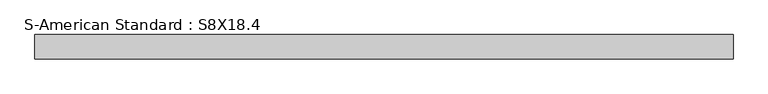
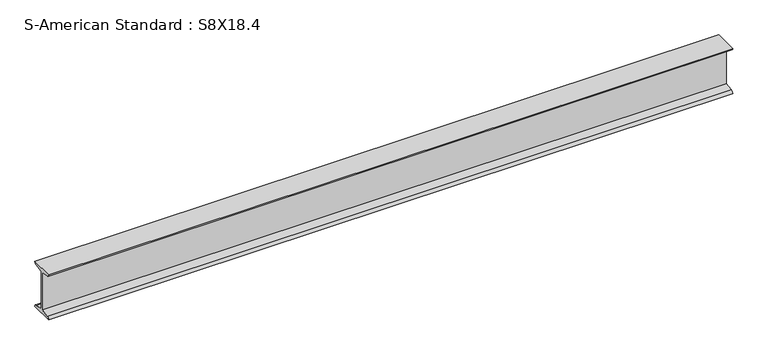
"""IFC4 building model written with IfcOpenShell, lengths in millimetres: beam geometry, S-American Standard : S8X18.4."""

from ifc_helpers import new_model, si_unit, point, frame, frame_2d, origin, place, context, project, spatial, polyline, circle_curve, trimmed, segment, composite_curve, outline, extrude, source, transform, mapped, element, save


def s_american_standard_s8x18_4_0708d1c2(model_context):
    return source(origin(), model_context, "Body", "SweptSolid", [
        extrude(outline(composite_curve([segment(polyline([(-50.8, 101.6), (50.8, 101.6)]), True, "CONTINUOUS"), segment(trimmed(circle_curve(frame_2d((40.005, 101.6)), 10.795), [point((50.8, 101.6))], [point((40.005, 90.805))], False, "CARTESIAN"), True, "CONTINUOUS"), segment(polyline([(40.005, 90.805), (3.4417, 85.0139422), (3.4417, -85.0139422), (40.005, -90.805)]), True, "CONTINUOUS"), segment(trimmed(circle_curve(frame_2d((40.005, -101.6)), 10.795), [point((40.005, -90.805))], [point((50.8, -101.6))], False, "CARTESIAN"), True, "CONTINUOUS"), segment(polyline([(50.8, -101.6), (-50.8, -101.6)]), True, "CONTINUOUS"), segment(trimmed(circle_curve(frame_2d((-40.005, -101.6)), 10.795), [point((-50.8, -101.6))], [point((-40.005, -90.805))], False, "CARTESIAN"), True, "CONTINUOUS"), segment(polyline([(-40.005, -90.805), (-3.4417, -85.0139422), (-3.4417, 85.0139422), (-40.005, 90.805)]), True, "CONTINUOUS"), segment(trimmed(circle_curve(frame_2d((-40.005, 101.6)), 10.795), [point((-40.005, 90.805))], [point((-50.8, 101.6))], False, "CARTESIAN"), True, "CONTINUOUS")], self_intersect=False)), frame((-1473.581, 0.0, 0.0), z_axis=(1.0, 0.0, 0.0), x_axis=(0.0, 1.0, 0.0)), (0.0, 0.0, 1.0), 2908.808),
    ])


if __name__ == "__main__":
    model = new_model("IFC4")
    model_context = context("Model", 3, world=origin())
    ifc_project = project(units=[si_unit("LENGTHUNIT", "METRE", prefix="MILLI")], contexts=[model_context])
    site = spatial("IfcSite", under=ifc_project)
    building = spatial("IfcBuilding", under=site)
    placement = place(None, origin())
    s_american_standard_s8x18_4_shape = s_american_standard_s8x18_4_0708d1c2(model_context)
    element("IfcBeam", 1, ObjectType="S-American Standard : S8X18.4", at=placement, inside=building, context=model_context, shape_type="MappedRepresentation", body=[
        mapped(s_american_standard_s8x18_4_shape, transform((0.0, 0.0, 0.0), x_axis=(1.0, 0.0, 0.0), y_axis=(0.0, 1.0, 0.0), z_axis=(0.0, 0.0, 1.0))),
    ])
    save(model, "model.ifc")

# Revit data of these elements
# Type "S-American Standard : S8X18.4"
#   Assembly Code = "B10"
#   W = 18.4
#   Length [instance default] = 5' - 0"
#   bf = 0' - 4"
#   d = 0' - 8"
#   k = 0' - 1"
#   tf = 0' - 0.425"
#   tw = 0' - 0.271"
#   A = 0.0375 SF
#   Structural Material [instance default] = Steel ASTM A572
# Element 1 (IfcBeam, "S-American Standard : S8X18.4")
#   Materials on its faces: "Steel ASTM A572"
# Materials
#   "Steel ASTM A572": class "Metal", colour RGB 247 247 247, transparency 0, Description = "Structural steel, high strength low alloy, ASTM - A572 - 50", Cost = 0
